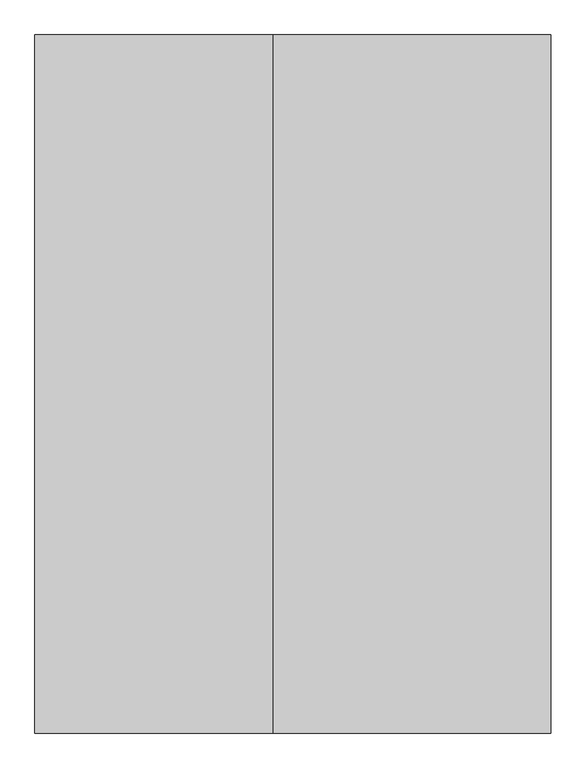
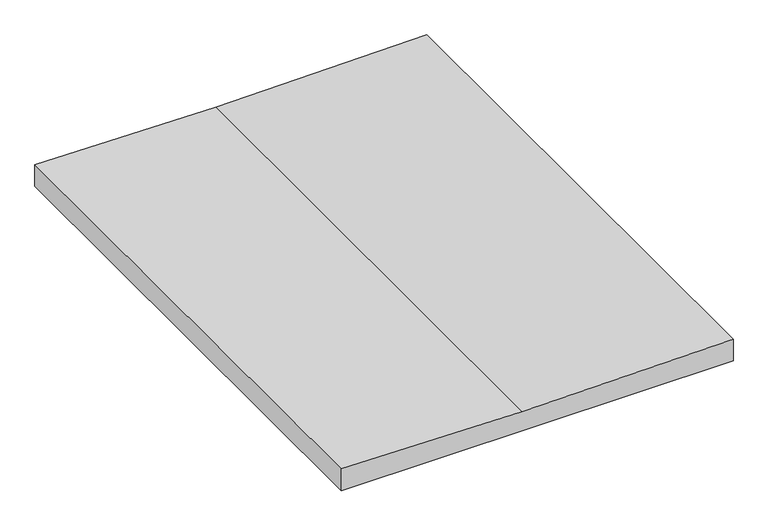
"""IFC4 building model written with IfcOpenShell, lengths in millimetres: proxy geometry, FIRESTONE INSULATION2:FIRESTONE INSULATION003:295699 : FIRESTONE INSULATION2:FIRESTONE INSULATION003:295699."""

from ifc_helpers import new_model, si_unit, frame, origin, place, context, project, spatial, polyline, outline, extrude, source, transform, mapped, element, save


def generic_models_fe95cb31(model_context):
    return source(origin(), model_context, "Body", "SweptSolid", [
        extrude(outline(polyline([(40218.4000089, 2209.6354065), (40131.746, 2209.6354065), (40131.746, 3686.9275669), (40218.4000089, 3686.9275669), (40208.6021556, 2890.4461596), (40218.4000089, 2209.6354065)])), frame((0.0, 1278.3325411, 0.0), z_axis=(0.0, 1.0, 0.0), x_axis=(0.0, 0.0, 1.0)), (0.0, 0.0, 1.0), 2000.0),
    ])


if __name__ == "__main__":
    model = new_model("IFC4")
    model_context = context("Model", 3, world=origin())
    ifc_project = project(units=[si_unit("LENGTHUNIT", "METRE", prefix="MILLI")], contexts=[model_context])
    site = spatial("IfcSite", under=ifc_project)
    building = spatial("IfcBuilding", under=site)
    placement = place(None, origin())
    generic_models_shape = generic_models_fe95cb31(model_context)
    element("IfcBuildingElementProxy", 1, Name="FIRESTONE INSULATION2:FIRESTONE INSULATION003:295699 : FIRESTONE INSULATION2:FIRESTONE INSULATION003:295699", ObjectType="FIRESTONE INSULATION2:FIRESTONE INSULATION003:295699 : FIRESTONE INSULATION2:FIRESTONE INSULATION003:295699", at=placement, inside=building, context=model_context, shape_type="MappedRepresentation", body=[
        mapped(generic_models_shape, transform((0.0, 0.0, 0.0), x_axis=(1.0, 0.0, 0.0), y_axis=(0.0, 1.0, 0.0), z_axis=(0.0, 0.0, 1.0))),
    ])
    save(model, "model.ifc")

# Revit data of these elements
# Type "FIRESTONE INSULATION2:FIRESTONE INSULATION003:295699 : FIRESTONE INSULATION2:FIRESTONE INSULATION003:295699"
#   NameOverride = "FIRESTONE INSULATION2:FIRESTONE INSULATION003:295699"
#   ObjectTypeOverride = "FIRESTONE INSULATION2:FIRESTONE INSULATION003"
#   Reference = "FIRESTONE INSULATION003"
#   Category = "Generic Models"
#   Tag = "295699"
# Element 1 (IfcBuildingElementProxy, "FIRESTONE INSULATION2:FIRESTONE INSULATION003:295699 : FIRESTONE INSULATION2:FIRESTONE INSULATION003:295699")
#   Materials on its faces: "TAPERED 2X SLEEPERS - SLOPED TO DRAIN"
# Materials
#   "TAPERED 2X SLEEPERS - SLOPED TO DRAIN": class "Unassigned", colour RGB 234 198 178, transparency 0
